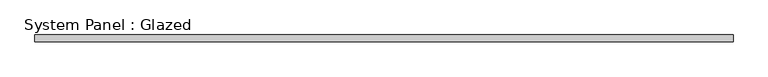
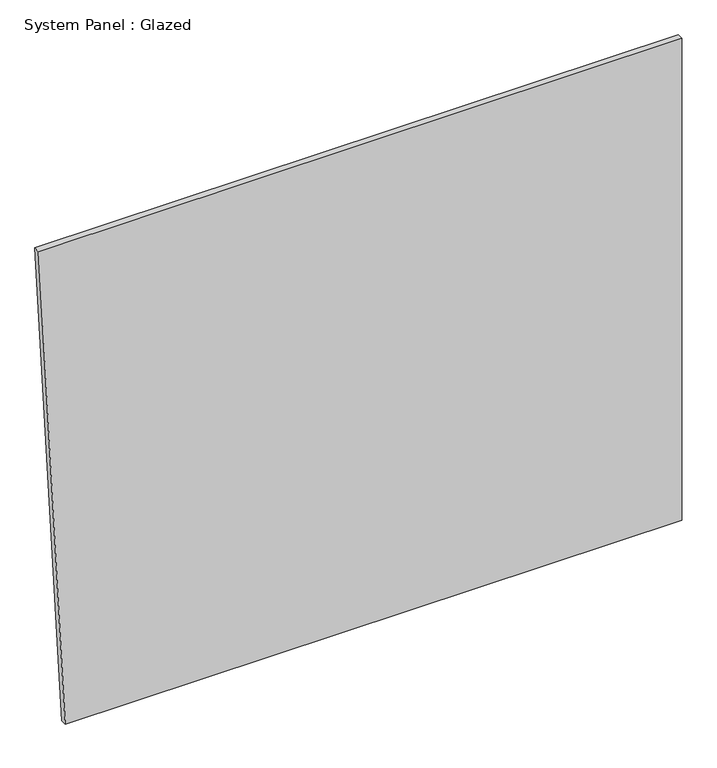
"""IFC4 building model written with IfcOpenShell, lengths in millimetres: plate geometry, System Panel : Glazed."""

from ifc_helpers import new_model, si_unit, frame, origin, place, context, project, spatial, polyline, outline, extrude, source, transform, mapped, element, save


def system_panel_glazed_e0da27cb(model_context):
    return source(origin(), model_context, "Body", "SweptSolid", [
        extrude(outline(polyline([(0.0, -1208.7338763), (0.0, 1317.8741594), (2085.3785982, 1317.8741594), (2085.3785982, -1317.8741594), (0.0, -1208.7338763)])), frame((0.0, -44.45, 0.0), z_axis=(0.0, 1.0, 0.0), x_axis=(0.0, 0.0, 1.0)), (0.0, 0.0, 1.0), 25.4),
    ])


if __name__ == "__main__":
    model = new_model("IFC4")
    model_context = context("Model", 3, world=origin())
    ifc_project = project(units=[si_unit("LENGTHUNIT", "METRE", prefix="MILLI")], contexts=[model_context])
    site = spatial("IfcSite", under=ifc_project)
    building = spatial("IfcBuilding", under=site)
    placement = place(None, origin())
    system_panel_glazed_shape = system_panel_glazed_e0da27cb(model_context)
    element("IfcPlate", 1, ObjectType="System Panel : Glazed", at=placement, inside=building, context=model_context, shape_type="MappedRepresentation", body=[
        mapped(system_panel_glazed_shape, transform((0.0, 0.0, 0.0), x_axis=(1.0, 0.0, 0.0), y_axis=(0.0, 1.0, 0.0), z_axis=(0.0, 0.0, 1.0))),
    ])
    save(model, "model.ifc")

# Revit data of these elements
# Type "System Panel : Glazed"
#   Construction Type Id = "GSP4R"
#   Analytic Construction = "1/8 in Pilkington single glazing"
#   Visual Light Transmittance = 0.9
#   Solar Heat Gain Coefficient = 0.86
#   Heat Transfer Coefficient (U) = 1.18115 BTU/(h·ft²·°F)
#   Define Thermal Properties by = 1
# Element 1 (IfcPlate, "System Panel : Glazed")
#   Materials on its faces: "Glass"
# Materials
#   "Glass": class "Glass", colour RGB 0 128 192, transparency 0.75, Description = "Soda Lime Glass", Cost = 0
